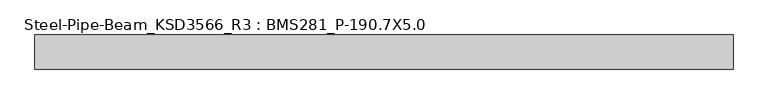
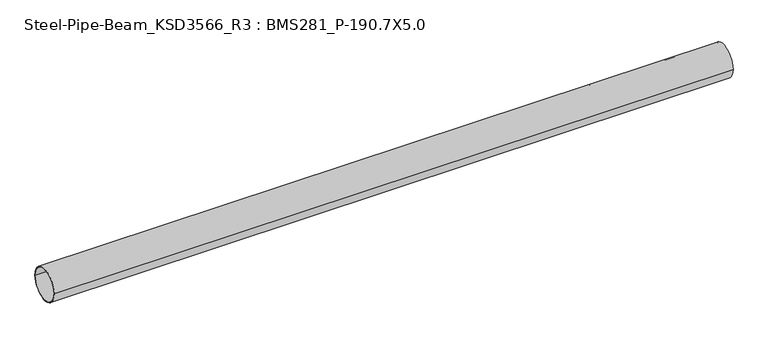
"""IFC4 building model written with IfcOpenShell, lengths in millimetres: member geometry, Steel-Pipe-Beam_KSD3566_R3 : BMS281_P-190.7X5.0."""

from ifc_helpers import new_model, si_unit, point, frame, origin, origin_2d, place, context, project, spatial, circle_curve, trimmed, segment, composite_curve, outline, extrude, source, transform, mapped, element, save


def steel_pipe_beam_ksd3566_r3_bms281_p_190_7x5_0_b4955ca0(model_context):
    return source(origin(), model_context, "Body", "SweptSolid", [
        extrude(outline(composite_curve([segment(trimmed(circle_curve(origin_2d(), 95.35), [point((95.35, 0.0))], [point((-95.35, 0.0))], False, "CARTESIAN"), True, "CONTINUOUS"), segment(trimmed(circle_curve(origin_2d(), 95.35), [point((-95.35, 0.0))], [point((95.35, 0.0))], False, "CARTESIAN"), True, "CONTINUOUS")], self_intersect=False), holes=[composite_curve([segment(trimmed(circle_curve(origin_2d(), 90.35), [point((-90.35, 0.0))], [point((90.35, 0.0))], True, "CARTESIAN"), True, "CONTINUOUS"), segment(trimmed(circle_curve(origin_2d(), 90.35), [point((90.35, 0.0))], [point((-90.35, 0.0))], True, "CARTESIAN"), True, "CONTINUOUS")], self_intersect=False)]), frame((-1965.4682703, 0.0, 0.0), z_axis=(1.0, 0.0, 0.0), x_axis=(0.0, 1.0, 0.0)), (0.0, 0.0, 1.0), 3898.3272248),
    ])


if __name__ == "__main__":
    model = new_model("IFC4")
    model_context = context("Model", 3, world=origin())
    ifc_project = project(units=[si_unit("LENGTHUNIT", "METRE", prefix="MILLI")], contexts=[model_context])
    site = spatial("IfcSite", under=ifc_project)
    building = spatial("IfcBuilding", under=site)
    placement = place(None, origin())
    steel_pipe_beam_ksd3566_r3_bms281_p_190_7x5_0_shape = steel_pipe_beam_ksd3566_r3_bms281_p_190_7x5_0_b4955ca0(model_context)
    element("IfcMember", 1, ObjectType="Steel-Pipe-Beam_KSD3566_R3 : BMS281_P-190.7X5.0", at=placement, inside=building, context=model_context, shape_type="MappedRepresentation", body=[
        mapped(steel_pipe_beam_ksd3566_r3_bms281_p_190_7x5_0_shape, transform((0.0, 0.0, 0.0), x_axis=(1.0, 0.0, 0.0), y_axis=(0.0, 1.0, 0.0), z_axis=(0.0, 0.0, 1.0))),
    ])
    save(model, "model.ifc")

# Revit data of these elements
# Type "Steel-Pipe-Beam_KSD3566_R3 : BMS281_P-190.7X5.0"
#   Keynote = "P-190.7X5.0"
#   SteelWeight = "Light"
#   t = 0.0050 m
#   Surface Area = 0.599102 m²/m
#   Section Area = 29.1697 cm²
#   Mass per Unit Length = 22.8982 kg/m
#   Length [instance default] = 1.5000 m
#   D = 0.1907 m
#   hec_material4 [instance default] = none
#   hec_material3 [instance default] = none
#   hec_material2 [instance default] = none
#   hec_material1 [instance default] = none
#   Structural Material [instance default] = Steel, 45-345
#   Assembly Code = ""
# Element 1 (IfcMember, "Steel-Pipe-Beam_KSD3566_R3 : BMS281_P-190.7X5.0")
#   Structural Material = none
# Materials
#   "Steel, 45-345": class "Metal", colour RGB 189 187 185, transparency 0, Description = "Steel 345 MPa", Cost = 0
